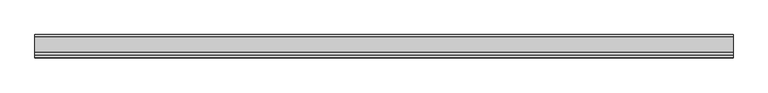
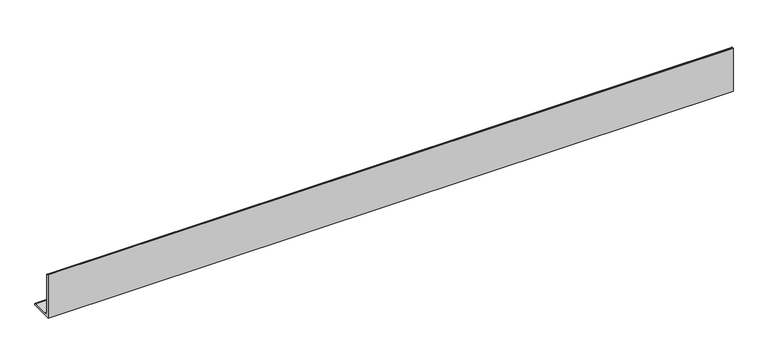
"""IFC4 building model written with IfcOpenShell, lengths in millimetres: beam geometry, NLRS_28_SF_LIB_stalen ligger hoekprofiel ongelijkzijdig-AV-MMBS-SRP_gen_rsf : stalen ligger ongelijzijdig hoekprofiel LUEQ_gen__200x100x10."""

from ifc_helpers import new_model, si_unit, point, frame, frame_2d, origin, place, context, project, spatial, polyline, circle_curve, trimmed, segment, composite_curve, outline, extrude, source, transform, mapped, element, save


def beam_ba2c4c4c(model_context):
    return source(origin(), model_context, "Body", "SweptSolid", [
        extrude(outline(composite_curve([segment(polyline([(-20.13, -69.3), (-20.13, 130.7), (-17.63, 130.7)]), True, "CONTINUOUS"), segment(trimmed(circle_curve(frame_2d((-17.63, 123.2)), 7.5), [point((-17.63, 130.7))], [point((-10.13, 123.2))], False, "CARTESIAN"), True, "CONTINUOUS"), segment(polyline([(-10.13, 123.2), (-10.13, -44.3)]), True, "CONTINUOUS"), segment(trimmed(circle_curve(frame_2d((4.87, -44.3)), 15.0), [point((-10.13, -44.3))], [point((4.87, -59.3))], True, "CARTESIAN"), True, "CONTINUOUS"), segment(polyline([(4.87, -59.3), (72.37, -59.3)]), True, "CONTINUOUS"), segment(trimmed(circle_curve(frame_2d((72.37, -66.8)), 7.5), [point((72.37, -59.3))], [point((79.87, -66.8))], False, "CARTESIAN"), True, "CONTINUOUS"), segment(polyline([(79.87, -66.8), (79.87, -69.3), (-20.13, -69.3)]), True, "CONTINUOUS")], self_intersect=False)), frame((-1500.0, 0.0, 0.0), z_axis=(1.0, 0.0, 0.0), x_axis=(0.0, 1.0, 0.0)), (0.0, 0.0, 1.0), 3000.0),
    ])


if __name__ == "__main__":
    model = new_model("IFC4")
    model_context = context("Model", 3, world=origin())
    ifc_project = project(units=[si_unit("LENGTHUNIT", "METRE", prefix="MILLI")], contexts=[model_context])
    site = spatial("IfcSite", under=ifc_project)
    building = spatial("IfcBuilding", under=site)
    placement = place(None, origin())
    beam_shape = beam_ba2c4c4c(model_context)
    element("IfcBeam", 1, ObjectType="NLRS_28_SF_LIB_stalen ligger hoekprofiel ongelijkzijdig-AV-MMBS-SRP_gen_rsf : stalen ligger ongelijzijdig hoekprofiel LUEQ_gen__200x100x10", at=placement, inside=building, context=model_context, shape_type="MappedRepresentation", body=[
        mapped(beam_shape, transform((0.0, 0.0, 0.0), x_axis=(1.0, 0.0, 0.0), y_axis=(0.0, 1.0, 0.0), z_axis=(0.0, 0.0, 1.0))),
    ])
    save(model, "model.ifc")

# Revit data of these elements
# Type "NLRS_28_SF_LIB_stalen ligger hoekprofiel ongelijkzijdig-AV-MMBS-SRP_gen_rsf : stalen ligger ongelijzijdig hoekprofiel LUEQ_gen__200x100x10"
#   Type IfcGUID = "0dxhH9VHH5jh7XQ0uLfXuR"
#   IfcExportAs = "IfcBeamType"
#   Type Comments = "L200x100x10"
#   Model = " "
#   Manufacturer = " "
#   Fire Rating = " "
#   Description = "stalen ligger L200x100x10"
#   Assembly Code = "28.11"
#   vz = 130.7 mm
#   vy = 79.87 mm
#   tw = 10 mm
#   tf = 10 mm
#   ri = 7.5 mm
#   ra = 15 mm
#   d = 200 mm
#   bf = 100 mm
#   NLRS_C_lengte [instance default] = 1524 mm
#   Length [instance default] = 1524 mm
#   Structural Material = NLRS_h2_staal_gen_rsf
#   Keynote = ""
# Element 1 (IfcBeam, "NLRS_28_SF_LIB_stalen ligger hoekprofiel ongelijkzijdig-AV-MMBS-SRP_gen_rsf : stalen ligger ongelijzijdig hoekprofiel LUEQ_gen__200x100x10")
#   NLRS_C_lengte = 3000 mm
#   Materials on its faces: "NLRS_h2_staal_gen_rsf"
# Materials
#   "NLRS_h2_staal_gen_rsf": class "H - Metaal", colour RGB 189 187 185, transparency 0, Keynote = "h2", Manufacturer = "Revit Standards Foundation", URL = "www.revitstandards.org", Description = "staal", Cost = 0
